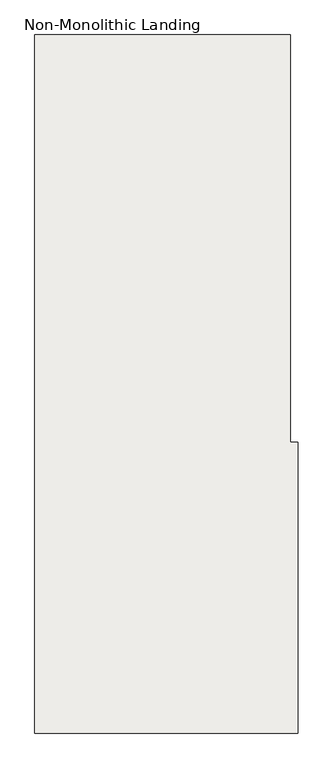
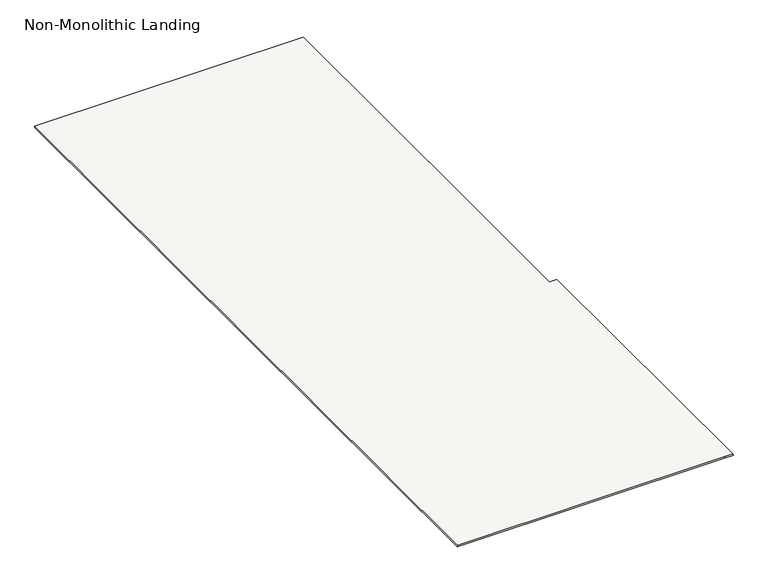
"""IFC4 building model written with IfcOpenShell, lengths in millimetres: slab geometry, Non-Monolithic Landing."""

from ifc_helpers import new_model, si_unit, origin, place, context, project, spatial, faceted_brep, source, transform, mapped, element, save


def non_monolithic_landing_72f17e9e(model_context):
    return source(origin(), model_context, "Body", "Brep", [
        faceted_brep([(13356.0599092, 10220.4345331, 16294.1176471), (13356.9099092, 10220.4345331, 16288.1176471), (13356.9099092, 11470.4345331, 16288.1176471), (13356.0599092, 11470.4345331, 16294.1176471), (13325.0, 13220.4345331, 16294.1176471), (12225.0, 13220.4345331, 16294.1176471), (12225.0, 10220.4345331, 16294.1176471), (13325.0, 10220.4345331, 16294.1176471), (13325.0, 11470.4345331, 16294.1176471), (13325.0, 12030.4345331, 16294.1176471), (12225.0, 10220.4345331, 16288.1176471), (12225.0, 13220.4345331, 16288.1176471), (13324.15, 13220.4345331, 16288.1176471), (13324.15, 12030.4345331, 16288.1176471), (13325.0, 12030.4345331, 16288.1176471), (13325.0, 11470.4345331, 16288.1176471), (13325.0, 10220.4345331, 16288.1176471)], [[[0, 1, 2, 3]], [[4, 5, 6, 7, 0, 3, 8, 9]], [[10, 11, 12, 13, 14, 15, 2, 1, 16]], [[9, 8, 15, 14]], [[0, 7, 16, 1]], [[7, 6, 10, 16]], [[6, 5, 11, 10]], [[5, 4, 12, 11]], [[13, 9, 14]], [[9, 13, 12, 4]], [[8, 3, 2, 15]]]),
    ])


if __name__ == "__main__":
    model = new_model("IFC4")
    model_context = context("Model", 3, world=origin())
    ifc_project = project(units=[si_unit("LENGTHUNIT", "METRE", prefix="MILLI")], contexts=[model_context])
    site = spatial("IfcSite", under=ifc_project)
    building = spatial("IfcBuilding", under=site)
    placement = place(None, origin())
    non_monolithic_landing_shape = non_monolithic_landing_72f17e9e(model_context)
    element("IfcSlab", 1, ObjectType="Non-Monolithic Landing", at=placement, inside=building, context=model_context, shape_type="MappedRepresentation", body=[
        mapped(non_monolithic_landing_shape, transform((0.0, 0.0, 0.0), x_axis=(1.0, 0.0, 0.0), y_axis=(0.0, 1.0, 0.0), z_axis=(0.0, 0.0, 1.0))),
    ])
    save(model, "model.ifc")

# Revit data of these elements
# Element 1 (IfcSlab, "Non-Monolithic Landing")
#   Materials on its faces: "Steel, Paint Finish, Dark Gray"
# Materials
#   "Steel, Paint Finish, Dark Gray": class "Metal", colour RGB 89 89 89, transparency 0, Description = "Steel, paint finish, dark gray, glossy", Cost = 0
